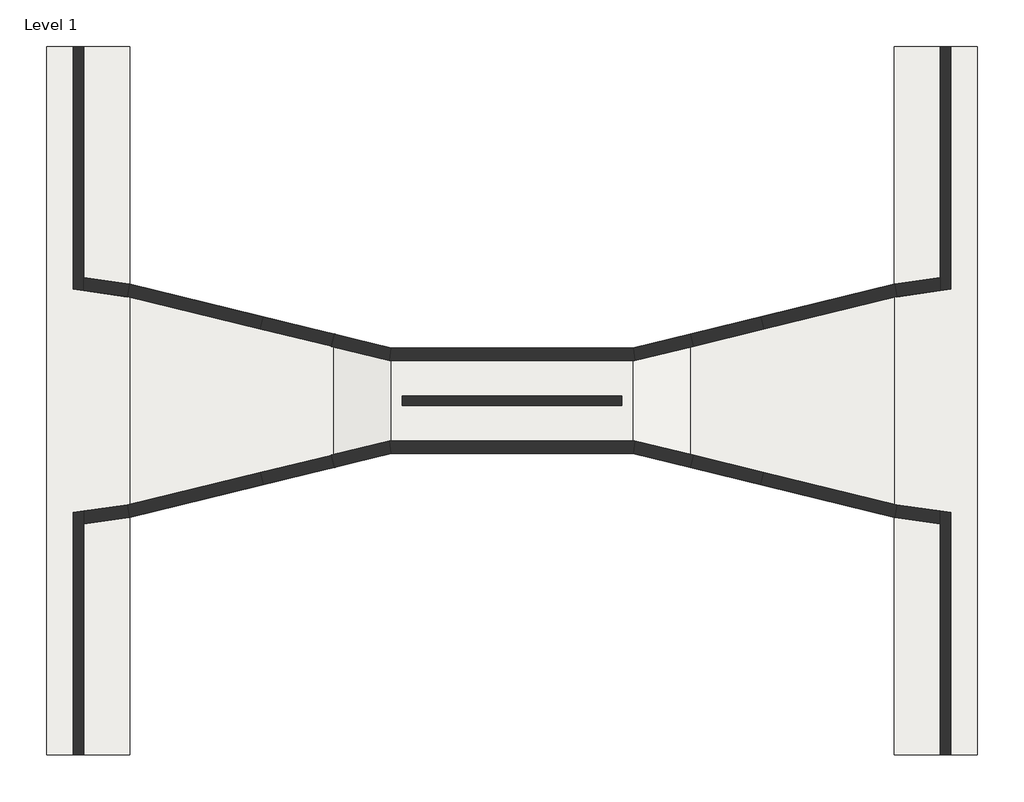
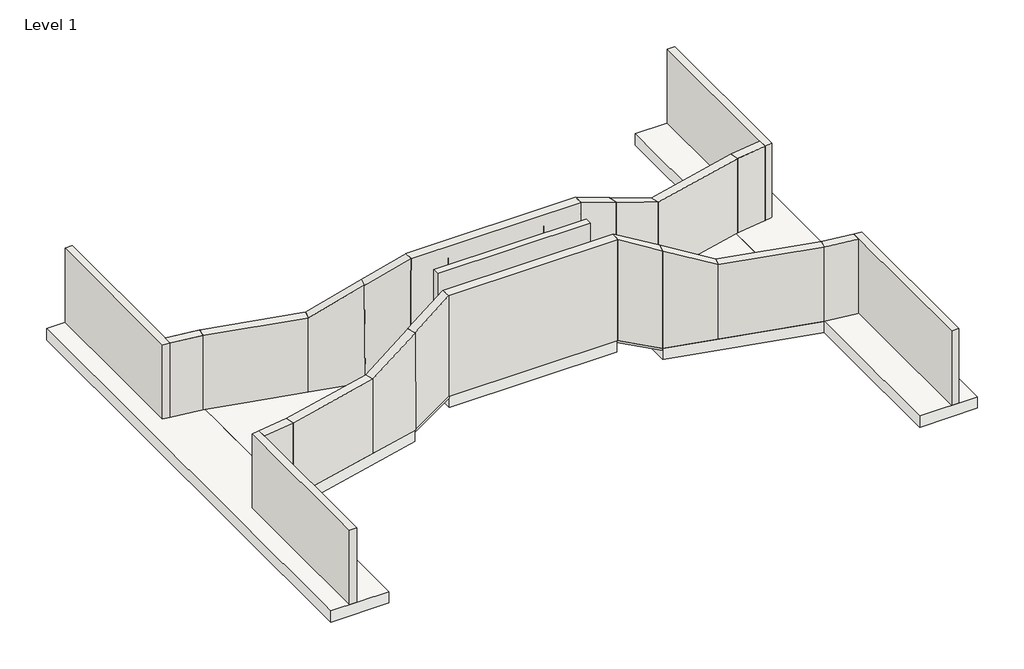
# One storey: 32 walls, 7 slabs.
"""IFC4 building model written with IfcOpenShell, lengths in millimetres."""

from ifc_helpers import new_model, si_unit, frame, origin, place, context, project, spatial, polyline, outline, extrude, faceted_brep, element, save

model = new_model("IFC4")

# Units and contexts
model_context = context("Model", 3, world=origin())
ifc_project = project(units=[si_unit("LENGTHUNIT", "METRE", prefix="MILLI")], contexts=[model_context])

# Site, building, storey
site = spatial("IfcSite", under=ifc_project)
building = spatial("IfcBuilding", under=site)
storey = spatial("IfcBuildingStorey", under=building, Name="Level 1", Elevation=0.0)

# Slabs
placement = place(None, origin())
element("IfcSlab", 1, ObjectType="Appronl", at=placement, inside=storey, context=model_context, shape_type="SweptSolid", body=[
    extrude(outline(polyline([(21800.0, -16601.0), (17901.0, -16601.0), (17901.0, 16601.0), (21800.0, 16601.0), (21800.0, -16601.0)])), frame((0.0, 0.0, -3600.0), z_axis=(0.0, 0.0, 1.0), x_axis=(1.0, 0.0, 0.0)), (0.0, 0.0, 1.0), 800.0),
])
element("IfcSlab", 2, ObjectType="Appronl", at=placement, inside=storey, context=model_context, shape_type="SweptSolid", body=[
    extrude(outline(polyline([(8350.0, 3127.0), (17901.0, 5458.0), (17901.0, -5458.0), (8350.0, -3127.0), (8350.0, 3127.0)])), frame((0.0, 0.0, -3600.0), z_axis=(0.0, 0.0, 1.0), x_axis=(1.0, 0.0, 0.0)), (0.0, 0.0, 1.0), 800.0),
])
element("IfcSlab", 3, ObjectType="Appronl", at=placement, inside=storey, context=model_context, shape_type="SweptSolid", body=[
    extrude(outline(polyline([(-21800.0, 16601.0), (-17901.0, 16601.0), (-17901.0, -16601.0), (-21800.0, -16601.0), (-21800.0, 16601.0)])), frame((0.0, 0.0, -3600.0), z_axis=(0.0, 0.0, 1.0), x_axis=(1.0, 0.0, 0.0)), (0.0, 0.0, 1.0), 800.0),
])
element("IfcSlab", 4, ObjectType="Appronl", at=placement, inside=storey, context=model_context, shape_type="SweptSolid", body=[
    extrude(outline(polyline([(-8350.0, 3127.0), (-8350.0, -3127.0), (-17901.0, -5458.0), (-17901.0, 5458.0), (-8350.0, 3127.0)])), frame((0.0, 0.0, -3600.0), z_axis=(0.0, 0.0, 1.0), x_axis=(1.0, 0.0, 0.0)), (0.0, 0.0, 1.0), 800.0),
])
element("IfcSlab", 5, ObjectType="Appronl", at=placement, inside=storey, context=model_context, shape_type="SweptSolid", body=[
    extrude(outline(polyline([(5650.0, 2468.0), (5650.0, -2468.0), (-5650.0, -2468.0), (-5650.0, 2468.0), (5650.0, 2468.0)])), frame((0.0, 0.0, -2500.0), z_axis=(0.0, 0.0, 1.0), x_axis=(1.0, 0.0, 0.0)), (0.0, 0.0, 1.0), 800.0),
])
element("IfcSlab", 6, ObjectType="3\" LW Concrete on 2\" Metal Deck", at=placement, inside=storey, context=model_context, shape_type="Brep", body=[
    faceted_brep([(-5650.0, 2468.0, -1837.1353501), (-5650.0, -2468.0, -1837.1353501), (-8350.0, -3127.0, -2937.1353501), (-8350.0, 3127.0, -2937.1353501), (-5650.0, 2468.0, -1700.0), (-8350.0, 3127.0, -2800.0), (-8350.0, -3127.0, -2800.0), (-5650.0, -2468.0, -1700.0)], [[[0, 1, 2, 3]], [[4, 5, 6, 7]], [[1, 0, 4, 7]], [[2, 1, 7, 6]], [[3, 2, 6, 5]], [[0, 3, 5, 4]]]),
])
element("IfcSlab", 7, ObjectType="3\" LW Concrete on 2\" Metal Deck", at=placement, inside=storey, context=model_context, shape_type="Brep", body=[
    faceted_brep([(5650.0, 2468.0, -1837.1353501), (8350.0, 3127.0, -2937.1353501), (8350.0, -3127.0, -2937.1353501), (5650.0, -2468.0, -1837.1353501), (5650.0, 2468.0, -1700.0), (5650.0, -2468.0, -1700.0), (8350.0, -3127.0, -2800.0), (8350.0, 3127.0, -2800.0)], [[[0, 1, 2, 3]], [[4, 5, 6, 7]], [[1, 0, 4, 7]], [[2, 1, 7, 6]], [[3, 2, 6, 5]], [[0, 3, 5, 4]]]),
])

# Walls
element("IfcWall", 8, ObjectType="Wingwall", at=placement, inside=storey, context=model_context, shape_type="SweptSolid", body=[
    extrude(outline(polyline([(-20050.0, 5767.2805137), (-17916.0428831, 5461.9054729), (-18029.9571169, 4872.0945271), (-20050.0, 5161.1681326), (-20050.0, 5767.2805137)])), frame((0.0, 0.0, -2800.0), z_axis=(0.0, 0.0, 1.0), x_axis=(1.0, 0.0, 0.0)), (0.0, 0.0, 1.0), 5300.0),
])
element("IfcWall", 9, ObjectType="Wingwall", at=placement, inside=storey, context=model_context, shape_type="SweptSolid", body=[
    extrude(outline(polyline([(-11792.4456337, 3349.3873565), (-18029.9571169, 4872.0945271), (-17916.0428831, 5461.9054729), (-11651.5543663, 3932.6126435), (-11792.4456337, 3349.3873565)])), frame((0.0, 0.0, -2800.0), z_axis=(0.0, 0.0, 1.0), x_axis=(1.0, 0.0, 0.0)), (0.0, 0.0, 1.0), 5300.0),
])
element("IfcWall", 10, ObjectType="Wingwall", at=placement, inside=storey, context=model_context, shape_type="Brep", body=[
    faceted_brep([(-11651.5543663, 3932.6126435, -2800.0), (-11651.5543663, 3932.6126435, 2500.3510698), (-8352.2565059, 3143.9904385, 4150.0), (-8280.2565059, 3126.780474, -2800.0), (-11792.4456336, 3349.3873565, -2800.0), (-8419.7434941, 2543.219526, -2800.0), (-8491.7434941, 2560.4294904, 4150.0), (-11792.4456336, 3349.3873565, 2499.6489302)], [[[0, 1, 2, 3]], [[4, 5, 6, 7]], [[2, 1, 7, 6]], [[3, 2, 6, 5]], [[0, 3, 5, 4]], [[1, 0, 4, 7]]]),
])
element("IfcWall", 11, ObjectType="Wingwall", at=placement, inside=storey, context=model_context, shape_type="Brep", body=[
    faceted_brep([(-8350.8659334, 3126.4445823, 4150.0), (-5685.9184792, 2476.0, 5482.4737271), (-5685.9184792, 2476.0, -1714.671918), (-8278.8659334, 3108.871249, -2800.0), (-8493.1340666, 2543.5554177, 4150.0), (-8421.1340666, 2525.9820843, -2800.0), (-5758.0815208, 1876.0, -1685.328082), (-5758.0815208, 1876.0, 5517.5262729)], [[[0, 1, 2, 3]], [[4, 5, 6, 7]], [[1, 0, 4, 7]], [[3, 2, 6, 5]], [[0, 3, 5, 4]], [[1, 7, 6, 2]]]),
])
element("IfcWall", 12, ObjectType="Wingwall", at=placement, inside=storey, context=model_context, shape_type="Brep", body=[
    faceted_brep([(5685.9184792, 2476.0, -1714.2806668), (5685.9184792, 2476.0, 5482.4737271), (8350.8659334, 3126.4445823, 4150.0), (8350.8659334, 3126.4445823, -2800.0), (5758.0815208, 1876.0, 5517.5262729), (5758.0815208, 1876.0, -1685.7193332), (8493.1340666, 2543.5554177, -2800.0), (8493.1340666, 2543.5554177, 4150.0)], [[[0, 1, 2, 3]], [[4, 5, 6, 7]], [[2, 1, 4, 7]], [[0, 3, 6, 5]], [[2, 7, 6, 3]], [[0, 5, 4, 1]]]),
])
element("IfcWall", 13, ObjectType="Wingwall", at=placement, inside=storey, context=model_context, shape_type="SweptSolid", body=[
    extrude(outline(polyline([(18029.9571169, 4872.0945271), (11793.1469574, 3349.5585643), (11650.8530426, 3932.4414357), (17916.0428831, 5461.9054729), (18029.9571169, 4872.0945271)])), frame((0.0, 0.0, -2800.0), z_axis=(0.0, 0.0, 1.0), x_axis=(1.0, 0.0, 0.0)), (0.0, 0.0, 1.0), 5300.0),
])
element("IfcWall", 14, ObjectType="Wingwall", at=placement, inside=storey, context=model_context, shape_type="SweptSolid", body=[
    extrude(outline(polyline([(17916.0428831, 5461.9054729), (20050.0, 5767.2805137), (20050.0, 5161.1681326), (18029.9571169, 4872.0945271), (17916.0428831, 5461.9054729)])), frame((0.0, 0.0, -2800.0), z_axis=(0.0, 0.0, 1.0), x_axis=(1.0, 0.0, 0.0)), (0.0, 0.0, 1.0), 5300.0),
])
element("IfcWall", 15, ObjectType="Wingwall", at=placement, inside=storey, context=model_context, shape_type="SweptSolid", body=[
    extrude(outline(polyline([(5300.0, 0.0), (6950.0, -3397.0039741), (0.0, -3397.0039741), (0.0, 0.0), (5300.0, 0.0)])), frame((11793.1803701, 3349.566723, -2800.0), z_axis=(-0.23726790022826785, 0.9714442565177216, 0.0), x_axis=(0.0, 0.0, 1.0)), (0.0, 0.0, 1.0), 600.0),
])
element("IfcWall", 16, ObjectType="Wingwall", at=placement, inside=storey, context=model_context, shape_type="SweptSolid", body=[
    extrude(outline(polyline([(-20050.0, -5161.1681326), (-18029.9571169, -4872.0945271), (-17916.0428831, -5461.9054729), (-20050.0, -5767.2805137), (-20050.0, -5161.1681326)])), frame((0.0, 0.0, -2800.0), z_axis=(0.0, 0.0, 1.0), x_axis=(1.0, 0.0, 0.0)), (0.0, 0.0, 1.0), 5300.0),
])
element("IfcWall", 17, ObjectType="Wingwall", at=placement, inside=storey, context=model_context, shape_type="SweptSolid", body=[
    extrude(outline(polyline([(-11651.5543663, -3932.6126435), (-17916.0428831, -5461.9054729), (-18029.9571169, -4872.0945271), (-11792.4456337, -3349.3873565), (-11651.5543663, -3932.6126435)])), frame((0.0, 0.0, -2800.0), z_axis=(0.0, 0.0, 1.0), x_axis=(1.0, 0.0, 0.0)), (0.0, 0.0, 1.0), 5300.0),
])
element("IfcWall", 18, ObjectType="Wingwall", at=placement, inside=storey, context=model_context, shape_type="Brep", body=[
    faceted_brep([(-11792.4456336, -3349.3873565, -2800.0), (-11792.4456336, -3349.3873565, 2499.6489302), (-8491.7434941, -2560.4294904, 4150.0), (-8419.7434941, -2543.219526, -2800.0), (-11651.5543663, -3932.6126435, -2800.0), (-8280.2565059, -3126.780474, -2800.0), (-8352.2565059, -3143.9904385, 4150.0), (-11651.5543663, -3932.6126435, 2500.3510698)], [[[0, 1, 2, 3]], [[4, 5, 6, 7]], [[2, 1, 7, 6]], [[3, 2, 6, 5]], [[0, 3, 5, 4]], [[1, 0, 4, 7]]]),
])
element("IfcWall", 19, ObjectType="Wingwall", at=placement, inside=storey, context=model_context, shape_type="Brep", body=[
    faceted_brep([(-8493.1340666, -2543.5554177, 4150.0), (-5758.0815208, -1876.0, 5517.5262729), (-5758.0815208, -1876.0, -1685.328082), (-8421.1340666, -2525.9820843, -2800.0), (-8350.8659334, -3126.4445823, 4150.0), (-8278.8659334, -3108.871249, -2800.0), (-5685.9184792, -2476.0, -1714.671918), (-5685.9184792, -2476.0, 5482.4737271)], [[[0, 1, 2, 3]], [[4, 5, 6, 7]], [[1, 0, 4, 7]], [[3, 2, 6, 5]], [[0, 3, 5, 4]], [[2, 1, 7, 6]]]),
])
element("IfcWall", 20, ObjectType="Wingwall", at=placement, inside=storey, context=model_context, shape_type="Brep", body=[
    faceted_brep([(5758.0815208, -1876.0, -1685.7193332), (5758.0815208, -1876.0, 5517.5262729), (8493.1340666, -2543.5554177, 4150.0), (8493.1340666, -2543.5554177, -2800.0), (5685.9184792, -2476.0, -1714.2806668), (8350.8659334, -3126.4445823, -2800.0), (8350.8659334, -3126.4445823, 4150.0), (5685.9184792, -2476.0, 5482.4737271)], [[[0, 1, 2, 3]], [[4, 5, 6, 7]], [[2, 1, 7, 6]], [[3, 2, 6, 5]], [[0, 3, 5, 4]], [[1, 0, 4, 7]]]),
])
element("IfcWall", 21, ObjectType="Wingwall", at=placement, inside=storey, context=model_context, shape_type="SweptSolid", body=[
    extrude(outline(polyline([(5300.0, 0.0), (6950.0, -3397.0039741), (0.0, -3397.0039741), (0.0, 0.0), (5300.0, 0.0)])), frame((11650.8196299, -3932.433277, -2800.0), z_axis=(0.23726790022826785, 0.9714442565177216, 0.0), x_axis=(0.0, 0.0, 1.0)), (0.0, 0.0, 1.0), 600.0),
])
element("IfcWall", 22, ObjectType="Wingwall", at=placement, inside=storey, context=model_context, shape_type="SweptSolid", body=[
    extrude(outline(polyline([(17916.0428831, -5461.9054729), (11650.8530426, -3932.4414357), (11793.1469574, -3349.5585643), (18029.9571169, -4872.0945271), (17916.0428831, -5461.9054729)])), frame((0.0, 0.0, -2800.0), z_axis=(0.0, 0.0, 1.0), x_axis=(1.0, 0.0, 0.0)), (0.0, 0.0, 1.0), 5300.0),
])
element("IfcWall", 23, ObjectType="Wingwall", at=placement, inside=storey, context=model_context, shape_type="SweptSolid", body=[
    extrude(outline(polyline([(18029.9571169, -4872.0945271), (20050.0, -5161.1681326), (20050.0, -5767.2805137), (17916.0428831, -5461.9054729), (18029.9571169, -4872.0945271)])), frame((0.0, 0.0, -2800.0), z_axis=(0.0, 0.0, 1.0), x_axis=(1.0, 0.0, 0.0)), (0.0, 0.0, 1.0), 5300.0),
])
element("IfcWall", 24, ObjectType="Wingwall", at=placement, inside=storey, context=model_context, shape_type="SweptSolid", body=[
    extrude(outline(polyline([(-20050.0, 5767.2805137), (-17930.5021265, 5463.9746298), (-18015.4978735, 4870.0253702), (-20050.0, 5161.1681326), (-20050.0, 5767.2805137)])), frame((0.0, 0.0, -2800.0), z_axis=(0.0, 0.0, 1.0), x_axis=(1.0, 0.0, 0.0)), (0.0, 0.0, 1.0), 5300.0),
])
element("IfcWall", 25, ObjectType="Wingwall", at=placement, inside=storey, context=model_context, shape_type="SweptSolid", body=[
    extrude(outline(polyline([(-11793.1469574, 3349.5585643), (-18029.9571169, 4872.0945271), (-17916.0428831, 5461.9054729), (-11650.8530426, 3932.4414357), (-11793.1469574, 3349.5585643)])), frame((0.0, 0.0, -2800.0), z_axis=(0.0, 0.0, 1.0), x_axis=(1.0, 0.0, 0.0)), (0.0, 0.0, 1.0), 5300.0),
])
element("IfcWall", 26, ObjectType="Wingwall", at=placement, inside=storey, context=model_context, shape_type="Brep", body=[
    faceted_brep([(-11651.5543663, 3932.6126435, -2800.0), (-11651.5543663, 3932.6126435, 2500.3510698), (-8352.2565059, 3143.9904385, 4150.0), (-8280.2565059, 3126.780474, -2800.0), (-11792.4456336, 3349.3873565, -2800.0), (-8419.7434941, 2543.219526, -2800.0), (-8491.7434941, 2560.4294904, 4150.0), (-11792.4456336, 3349.3873565, 2499.6489302)], [[[0, 1, 2, 3]], [[4, 5, 6, 7]], [[2, 1, 7, 6]], [[3, 2, 6, 5]], [[0, 3, 5, 4]], [[1, 0, 4, 7]]]),
])
element("IfcWall", 27, ObjectType="Wingwall", at=placement, inside=storey, context=model_context, shape_type="Brep", body=[
    faceted_brep([(-8350.8659334, 3126.4445823, 4150.0), (-5685.9184792, 2476.0, 5482.4737271), (-5685.9184792, 2476.0, -1714.671918), (-8278.8659334, 3108.871249, -2800.0), (-8493.1340666, 2543.5554177, 4150.0), (-8421.1340666, 2525.9820843, -2800.0), (-5758.0815208, 1876.0, -1685.328082), (-5758.0815208, 1876.0, 5517.5262729)], [[[0, 1, 2, 3]], [[4, 5, 6, 7]], [[1, 0, 4, 7]], [[3, 2, 6, 5]], [[0, 3, 5, 4]], [[1, 7, 6, 2]]]),
])
element("IfcWall", 28, ObjectType="Wingwall", at=placement, inside=storey, context=model_context, shape_type="Brep", body=[
    faceted_brep([(5685.9184792, 2476.0, -1714.2806668), (5685.9184792, 2476.0, 5482.4737271), (8350.8659334, 3126.4445823, 4150.0), (8350.8659334, 3126.4445823, -2800.0), (5758.0815208, 1876.0, 5517.5262729), (5758.0815208, 1876.0, -1685.7193332), (8493.1340666, 2543.5554177, -2800.0), (8493.1340666, 2543.5554177, 4150.0)], [[[0, 1, 2, 3]], [[4, 5, 6, 7]], [[2, 1, 4, 7]], [[0, 3, 6, 5]], [[0, 5, 4, 1]], [[2, 7, 6, 3]]]),
])
element("IfcWall", 29, ObjectType="Wingwall", at=placement, inside=storey, context=model_context, shape_type="SweptSolid", body=[
    extrude(outline(polyline([(5300.0, 0.0), (6950.0, -3397.0039741), (0.0, -3397.0039741), (0.0, 0.0), (5300.0, 0.0)])), frame((11793.1803701, 3349.566723, -2800.0), z_axis=(-0.23726790022826785, 0.9714442565177216, 0.0), x_axis=(0.0, 0.0, 1.0)), (0.0, 0.0, 1.0), 600.0),
])
element("IfcWall", 30, ObjectType="Wingwall", at=placement, inside=storey, context=model_context, shape_type="SweptSolid", body=[
    extrude(outline(polyline([(18029.9571169, 4872.0945271), (11793.1469574, 3349.5585643), (11650.8530426, 3932.4414357), (17916.0428831, 5461.9054729), (18029.9571169, 4872.0945271)])), frame((0.0, 0.0, -2800.0), z_axis=(0.0, 0.0, 1.0), x_axis=(1.0, 0.0, 0.0)), (0.0, 0.0, 1.0), 5300.0),
])
element("IfcWall", 31, ObjectType="Wingwall", at=placement, inside=storey, context=model_context, shape_type="SweptSolid", body=[
    extrude(outline(polyline([(17930.5021265, 5463.9746298), (20050.0, 5767.2805137), (20050.0, 5161.1681326), (18015.4978735, 4870.0253702), (17930.5021265, 5463.9746298)])), frame((0.0, 0.0, -2800.0), z_axis=(0.0, 0.0, 1.0), x_axis=(1.0, 0.0, 0.0)), (0.0, 0.0, 1.0), 5300.0),
])
element("IfcWall", 32, ObjectType="Abutment", at=placement, inside=storey, context=model_context, shape_type="Brep", body=[
    faceted_brep([(-5758.0815208, 1876.0, -1700.0), (5758.0815208, 1876.0, -1700.0), (5758.0815208, 1876.0, 4673.4903305), (5722.0, 1876.0, 4673.4903305), (5722.0, 1876.0, 5500.0), (-5722.0, 1876.0, 5500.0), (-5722.0, 1876.0, 4673.4903305), (-5758.0815208, 1876.0, 4673.4903305), (-5685.9184792, 2476.0, -1700.0), (-5685.9184792, 2476.0, 4673.4903305), (-5722.0, 2476.0, 4673.4903305), (-5722.0, 2476.0, 5500.0), (5722.0, 2476.0, 5500.0), (5722.0, 2476.0, 4673.4903305), (5685.9184792, 2476.0, 4673.4903305), (5685.9184792, 2476.0, -1700.0), (-5722.0, 2176.0, 4673.4903305), (5722.0, 2176.0, 4673.4903305)], [[[0, 1, 2, 3, 4, 5, 6, 7]], [[8, 9, 10, 11, 12, 13, 14, 15]], [[1, 0, 8, 15]], [[5, 4, 12, 11]], [[6, 5, 11, 10, 16]], [[6, 16, 7]], [[0, 7, 16, 9, 8]], [[16, 10, 9]], [[4, 3, 17, 13, 12]], [[13, 17, 14]], [[2, 1, 15, 14, 17]], [[17, 3, 2]]]),
])
element("IfcWall", 33, ObjectType="Abutment", at=placement, inside=storey, context=model_context, shape_type="SweptSolid", body=[
    extrude(outline(polyline([(5685.9184792, -2476.0), (-5685.9184792, -2476.0), (-5758.0815208, -1876.0), (5758.0815208, -1876.0), (5685.9184792, -2476.0)])), frame((0.0, 0.0, -1700.0), z_axis=(0.0, 0.0, 1.0), x_axis=(1.0, 0.0, 0.0)), (0.0, 0.0, 1.0), 7200.0),
])
element("IfcWall", 34, ObjectType="Abutment", at=placement, inside=storey, context=model_context, shape_type="Brep", body=[
    faceted_brep([(-3227.648373, 1876.0, -1700.0), (3227.648373, 1876.0, -1700.0), (3227.648373, 1876.0, 4673.4903305), (5722.0, 1876.0, 4673.4903305), (5722.0, 1876.0, 5500.0), (-5722.0, 1876.0, 5500.0), (-5722.0, 1876.0, 4673.4903305), (-3227.648373, 1876.0, 4673.4903305), (-5685.9184792, 2476.0, -1700.0), (-5685.9184792, 2476.0, 4673.4903305), (-5722.0, 2476.0, 4673.4903305), (-5722.0, 2476.0, 5500.0), (5722.0, 2476.0, 5500.0), (5722.0, 2476.0, 4673.4903305), (5685.9184792, 2476.0, 4673.4903305), (5685.9184792, 2476.0, -1700.0)], [[[0, 1, 2, 3, 4, 5, 6, 7]], [[8, 9, 10, 11, 12, 13, 14, 15]], [[1, 0, 8, 15]], [[5, 4, 12, 11]], [[6, 5, 11, 10]], [[6, 10, 9, 7]], [[0, 7, 9, 8]], [[4, 3, 13, 12]], [[13, 3, 2, 14]], [[2, 1, 15, 14]]]),
])
element("IfcWall", 35, ObjectType="Pier", at=placement, inside=storey, context=model_context, shape_type="SweptSolid", body=[
    extrude(outline(polyline([(5150.0, -225.0), (-5150.0, -225.0), (-5150.0, 225.0), (5150.0, 225.0), (5150.0, -225.0)])), frame((0.0, 0.0, -1700.0), z_axis=(0.0, 0.0, 1.0), x_axis=(1.0, 0.0, 0.0)), (0.0, 0.0, 1.0), 7200.0),
])
element("IfcWall", 36, ObjectType="Return Wall", at=placement, inside=storey, context=model_context, shape_type="Brep", body=[
    faceted_brep([(20550.0, 5232.7194863, -2800.0), (20550.0, 16601.0, -2800.0), (20550.0, 16601.0, 2500.0), (20550.0, 5232.7194863, 2500.0), (20050.0, 5161.1681326, -2800.0), (20050.0, 5161.1681326, 2500.0), (20050.0, 5767.2805137, 2500.0), (20050.0, 16601.0, 2500.0), (20050.0, 16601.0, -2800.0), (20050.0, 5767.2805137, -2800.0)], [[[0, 1, 2, 3]], [[4, 5, 6, 7, 8, 9]], [[1, 0, 4, 9, 8]], [[2, 1, 8, 7]], [[3, 2, 7, 6, 5]], [[0, 3, 5, 4]]]),
])
element("IfcWall", 37, ObjectType="Return Wall", at=placement, inside=storey, context=model_context, shape_type="Brep", body=[
    faceted_brep([(20550.0, -16601.0, -2800.0), (20550.0, -5232.7194863, -2800.0), (20550.0, -5232.7194863, 2500.0), (20550.0, -16601.0, 2500.0), (20050.0, -16601.0, -2800.0), (20050.0, -16601.0, 2500.0), (20050.0, -5767.2805137, 2500.0), (20050.0, -5161.1681326, 2500.0), (20050.0, -5161.1681326, -2800.0), (20050.0, -5767.2805137, -2800.0)], [[[0, 1, 2, 3]], [[4, 5, 6, 7, 8, 9]], [[1, 0, 4, 9, 8]], [[3, 2, 7, 6, 5]], [[0, 3, 5, 4]], [[2, 1, 8, 7]]]),
])
element("IfcWall", 38, ObjectType="Return Wall", at=placement, inside=storey, context=model_context, shape_type="Brep", body=[
    faceted_brep([(-20050.0, -16601.0, -2800.0), (-20050.0, -5767.2805137, -2800.0), (-20050.0, -5161.1681326, -2800.0), (-20050.0, -5161.1681326, 2500.0), (-20050.0, -5767.2805137, 2500.0), (-20050.0, -16601.0, 2500.0), (-20550.0, -16601.0, -2800.0), (-20550.0, -16601.0, 2500.0), (-20550.0, -5232.7194863, 2500.0), (-20550.0, -5232.7194863, -2800.0)], [[[0, 1, 2, 3, 4, 5]], [[6, 7, 8, 9]], [[2, 1, 0, 6, 9]], [[5, 4, 3, 8, 7]], [[0, 5, 7, 6]], [[3, 2, 9, 8]]]),
])
element("IfcWall", 39, ObjectType="Return Wall", at=placement, inside=storey, context=model_context, shape_type="Brep", body=[
    faceted_brep([(-20050.0, 5161.1681326, -2800.0), (-20050.0, 5767.2805137, -2800.0), (-20050.0, 16601.0, -2800.0), (-20050.0, 16601.0, 2500.0), (-20050.0, 5767.2805137, 2500.0), (-20050.0, 5161.1681326, 2500.0), (-20550.0, 5232.7194863, -2800.0), (-20550.0, 5232.7194863, 2500.0), (-20550.0, 16601.0, 2500.0), (-20550.0, 16601.0, -2800.0)], [[[0, 1, 2, 3, 4, 5]], [[6, 7, 8, 9]], [[2, 1, 0, 6, 9]], [[3, 2, 9, 8]], [[5, 4, 3, 8, 7]], [[0, 5, 7, 6]]]),
])

save(model, "model.ifc")

# Revit data of these elements
# Project information
#   Project Issue Date = "Issue Date"
#   Project Status = "Project Status"
#   Client Name = "Owner"
#   Project Address = "Enter address here"
#   Project Name = "Project Name"
#   Project Number = "Project Number"
# Type "Appronl"
#   Assembly Code = "B1010"
#   Function = 0
#   Layers, outside or top first: 2' - 7.49606" "CONCR" (function 1)
# Type "3\" LW Concrete on 2\" Metal Deck"
#   Assembly Code = "B1010"
#   Function = 0
#   Layers, outside or top first: 0' - 5" "Concrete, Lightweight - 4 ksi" (function 1); 0' - 0" "Metal Deck" (function 200)
# Type "Wingwall"
#   Assembly Code = "B2010"
#   Layers, outside or top first: 1' - 11.62205" "CONCR" (function 1)
# Type "Abutment"
#   Assembly Code = "B2010"
#   Layers, outside or top first: 1' - 11.62205" "CONCR" (function 1)
# Type "Pier"
#   Assembly Code = "B2010"
#   Layers, outside or top first: 1' - 5.71654" "CONCR" (function 1)
# Type "Return Wall"
#   Assembly Code = "B2010"
#   Layers, outside or top first: 1' - 7.68504" "CONCR" (function 1)
# Elements 1, 2, 3, 4 (IfcSlab, "Appronl")
#   Height Offset From Level = -9' - 2.23622"
#   built-in parameter 1001954 = 1
#   Phase Created = New Construction
#   Materials on its faces: "CONCR"
# Element 5 (IfcSlab, "Appronl")
#   Height Offset From Level = -5' - 6.92913"
#   built-in parameter 1001954 = 1
#   Phase Created = New Construction
#   Materials on its faces: "CONCR"
# Elements 6, 7 (IfcSlab, "3\" LW Concrete on 2\" Metal Deck")
#   Height Offset From Level = -9' - 2.23622"
#   built-in parameter 1001954 = 1
#   Phase Created = New Construction
#   Materials on its faces: "Metal Deck", "Concrete, Lightweight - 4 ksi"
# Elements 8, 9, 13, 14, 16, 17, 22, 23, 24, 25, 30, 31 (IfcWall, "Wingwall")
#   built-in parameter 1001111 = -9' - 2.23622"
#   Top Offset = -1' - 9.5748"
#   Base Offset = -9' - 2.23622"
#   Unconnected Height = 17' - 4.66142"
#   wall height = 17' - 4.66142"
#   Phase Created = New Construction
#   Base Constraint = Level 1
#   Top Constraint = Level 2
#   Materials on its faces: "CONCR"
# Elements 10, 15, 18, 21, 26, 29 (IfcWall, "Wingwall")
#   built-in parameter 1001111 = -9' - 2.23622"
#   Top Offset = 3' - 7.38583"
#   Base Offset = -9' - 2.23622"
#   Unconnected Height = 22' - 9.62205"
#   wall height = 22' - 9.62205"
#   Phase Created = New Construction
#   Base Constraint = Level 1
#   Top Constraint = Level 2
#   Materials on its faces: "CONCR"
# Elements 11, 12, 19, 20, 27, 28 (IfcWall, "Wingwall")
#   built-in parameter 1001111 = -9' - 2.23622"
#   Top Offset = 8' - 0.53543"
#   Base Offset = -9' - 2.23622"
#   Unconnected Height = 27' - 2.77165"
#   wall height = 27' - 2.77165"
#   Phase Created = New Construction
#   Base Constraint = Level 1
#   Top Constraint = Level 2
#   Materials on its faces: "CONCR"
# Elements 32, 33, 34 (IfcWall, "Abutment")
#   built-in parameter 1001111 = -5' - 6.92913"
#   Top Offset = 8' - 0.53543"
#   Base Offset = -5' - 6.92913"
#   Unconnected Height = 23' - 7.46457"
#   wall height = 23' - 7.46457"
#   Phase Created = New Construction
#   Base Constraint = Level 1
#   Top Constraint = Level 2
#   Materials on its faces: "CONCR"
# Element 35 (IfcWall, "Pier")
#   built-in parameter 1001111 = -5' - 6.92913"
#   Top Offset = 8' - 0.53543"
#   Base Offset = -5' - 6.92913"
#   Unconnected Height = 23' - 7.46457"
#   wall height = 23' - 7.46457"
#   Phase Created = New Construction
#   Base Constraint = Level 1
#   Top Constraint = Level 2
#   Materials on its faces: "CONCR"
# Elements 36, 37, 38, 39 (IfcWall, "Return Wall")
#   built-in parameter 1001111 = -9' - 2.23622"
#   Top Offset = -1' - 9.5748"
#   Base Offset = -9' - 2.23622"
#   Unconnected Height = 17' - 4.66142"
#   wall height = 17' - 4.66142"
#   Phase Created = New Construction
#   Base Constraint = Level 1
#   Top Constraint = Level 2
#   Materials on its faces: "CONCR"
# Materials
#   "CONCR": class "Unassigned", colour RGB 192 192 192, transparency 0
#   "Concrete, Lightweight - 4 ksi": class "Concrete", colour RGB 127 127 127, transparency 0, Description = "Lightweight concrete 4 ksi", Cost = 0
#   "Metal Deck": class "Metal", colour RGB 199 199 199, transparency 0, Description = "Steel, mill finish", Cost = 0
